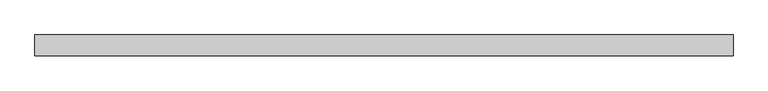
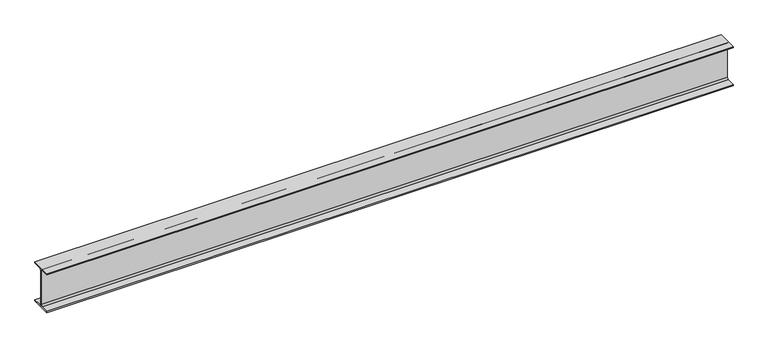
"""IFC4 building model written with IfcOpenShell, lengths in millimetres: beam geometry, 0912_Steel Framing_H-KSD3502 : H_SB_ASB_H-350x175x7x11."""

from ifc_helpers import new_model, si_unit, point, frame, frame_2d, origin, place, context, project, spatial, polyline, circle_curve, trimmed, segment, composite_curve, outline, extrude, source, transform, mapped, element, save


def beam_b071fafb(model_context):
    return source(origin(), model_context, "Body", "SweptSolid", [
        extrude(outline(composite_curve([segment(polyline([(87.5, -164.0), (87.5, -175.0), (-87.5, -175.0), (-87.5, -164.0), (-17.5, -164.0)]), True, "CONTINUOUS"), segment(trimmed(circle_curve(frame_2d((-17.5, -150.0)), 14.0), [point((-17.5, -164.0))], [point((-3.5, -150.0))], True, "CARTESIAN"), True, "CONTINUOUS"), segment(polyline([(-3.5, -150.0), (-3.5, 150.0)]), True, "CONTINUOUS"), segment(trimmed(circle_curve(frame_2d((-17.5, 150.0)), 14.0), [point((-3.5, 150.0))], [point((-17.5, 164.0))], True, "CARTESIAN"), True, "CONTINUOUS"), segment(polyline([(-17.5, 164.0), (-87.5, 164.0), (-87.5, 175.0), (87.5, 175.0), (87.5, 164.0), (17.5, 164.0)]), True, "CONTINUOUS"), segment(trimmed(circle_curve(frame_2d((17.5, 150.0)), 14.0), [point((17.5, 164.0))], [point((3.5, 150.0))], True, "CARTESIAN"), True, "CONTINUOUS"), segment(polyline([(3.5, 150.0), (3.5, -150.0)]), True, "CONTINUOUS"), segment(trimmed(circle_curve(frame_2d((17.5, -150.0)), 14.0), [point((3.5, -150.0))], [point((17.5, -164.0))], True, "CARTESIAN"), True, "CONTINUOUS"), segment(polyline([(17.5, -164.0), (87.5, -164.0)]), True, "CONTINUOUS")], self_intersect=False)), frame((-2920.1721181, 0.0, 0.0), z_axis=(1.0, 0.0, 0.0), x_axis=(0.0, 1.0, 0.0)), (0.0, 0.0, 1.0), 5810.1548079),
    ])


if __name__ == "__main__":
    model = new_model("IFC4")
    model_context = context("Model", 3, world=origin())
    ifc_project = project(units=[si_unit("LENGTHUNIT", "METRE", prefix="MILLI")], contexts=[model_context])
    site = spatial("IfcSite", under=ifc_project)
    building = spatial("IfcBuilding", under=site)
    placement = place(None, origin())
    beam_shape = beam_b071fafb(model_context)
    element("IfcBeam", 1, ObjectType="0912_Steel Framing_H-KSD3502 : H_SB_ASB_H-350x175x7x11", at=placement, inside=building, context=model_context, shape_type="MappedRepresentation", body=[
        mapped(beam_shape, transform((0.0, 0.0, 0.0), x_axis=(1.0, 0.0, 0.0), y_axis=(0.0, 1.0, 0.0), z_axis=(0.0, 0.0, 1.0))),
    ])
    save(model, "model.ifc")

# Revit data of these elements
# Type "0912_Steel Framing_H-KSD3502 : H_SB_ASB_H-350x175x7x11"
#   H_WM Code_1 = "S01AA002-00001 | Main Steel Structure Fabrication Work | Shelter/Building | Medium Steel - Standard (90KG/M>Weight≥30KG/M) | Material: (   )"
#   H_WM Code_2 = "S03AA028-00001 | Main Steel Structure Erection Work | Shelter/Building | Medium Steel (90KG/M>Weight≥30KG/M) | Material: (   )"
#   H_WM Code_3 = "S01AA010-00001 | Main Steel Structure Fabrication Work | Shelter/Building | Steel Painting/Coating | for Non-Fireproofed Steel Surface, Surface Preparation, Primer, Second & Final Coat | Material: (   )"
#   H_Q'ty Cal Type Tag = "SB-Q2"
#   Width = 17.5 cm
#   Web Thickness = 0.7 cm
#   Web Fillet = 1.4 cm
#   Warping Constant = 282000.0 cm⁶
#   W = 0
#   Torsional Moment of Inertia = 19.4042 cm⁴
#   Section Area = 63.14 cm²
#   Plastic Modulus weak axis = 174.0 cm³
#   Plastic Modulus strong axis = 868.0 cm³
#   Perimeter = 1.36 m²/m
#   Nominal Weight = 49.60 kgf/m
#   Moment of Inertia weak axis = 984.00 cm⁴
#   Moment of Inertia strong axis = 13600.00 cm⁴
#   Height = 35.0 cm
#   Flange Thickness = 1.1 cm
#   Elastic Modulus weak axis = 112.0 cm³
#   Elastic Modulus strong axis = 775.0 cm³
#   Centroid Vertical = 17.5 cm
#   Centroid Horizontal = 8.75 cm
#   Ix = 136000000
#   Length [instance default] = 1.5240 m
#   Zx = 868000
#   b = 0.1750 m
#   h = 0.3500 m
#   r = 0.0140 m
#   s = 0.0070 m
#   t = 0.0110 m
#   A = 0.006314 m²
#   Structural Material [instance default] = Steel, 45-345
#   Assembly Code = ""
# Element 1 (IfcBeam, "0912_Steel Framing_H-KSD3502 : H_SB_ASB_H-350x175x7x11")
#   Structural Material = none
# Materials
#   "Steel, 45-345": class "Metal", colour RGB 189 187 185, transparency 0, Description = "Steel 345 MPa", Cost = 0
